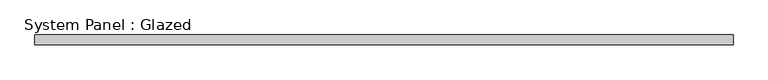
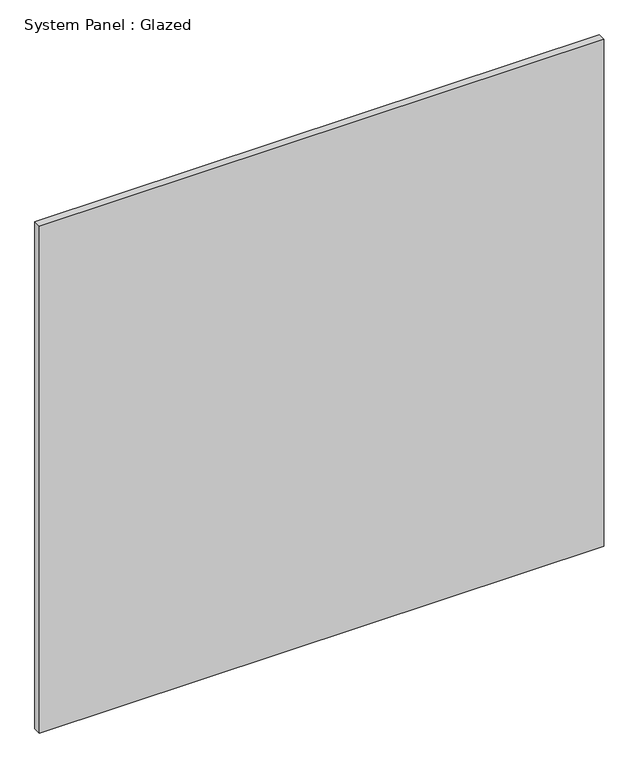
"""IFC4 building model written with IfcOpenShell, lengths in millimetres: plate geometry, System Panel : Glazed."""

from ifc_helpers import new_model, si_unit, origin, origin_with_axes, place, context, project, spatial, polyline, outline, extrude, source, transform, mapped, element, save


def system_panel_glazed_851df1f7(model_context):
    return source(origin(), model_context, "Body", "SweptSolid", [
        extrude(outline(polyline([(890.0000002, 24.5), (-890.0000002, 24.5), (-890.0000002, 49.5), (890.0000002, 49.5), (890.0000002, 24.5)])), origin_with_axes(), (0.0, 0.0, 1.0), 1690.2939092),
    ])


if __name__ == "__main__":
    model = new_model("IFC4")
    model_context = context("Model", 3, world=origin())
    ifc_project = project(units=[si_unit("LENGTHUNIT", "METRE", prefix="MILLI")], contexts=[model_context])
    site = spatial("IfcSite", under=ifc_project)
    building = spatial("IfcBuilding", under=site)
    placement = place(None, origin())
    system_panel_glazed_shape = system_panel_glazed_851df1f7(model_context)
    element("IfcPlate", 1, ObjectType="System Panel : Glazed", at=placement, inside=building, context=model_context, shape_type="MappedRepresentation", body=[
        mapped(system_panel_glazed_shape, transform((0.0, 0.0, 0.0), x_axis=(1.0, 0.0, 0.0), y_axis=(0.0, 1.0, 0.0), z_axis=(0.0, 0.0, 1.0))),
    ])
    save(model, "model.ifc")

# Revit data of these elements
# Element 1 (IfcPlate, "System Panel : Glazed")
#   Materials on its faces: "Glass"
# Materials
#   "Glass": class "Glass", colour RGB 218 227 224, transparency 0.85, Description = "Soda Lime Glass", Cost = 0
